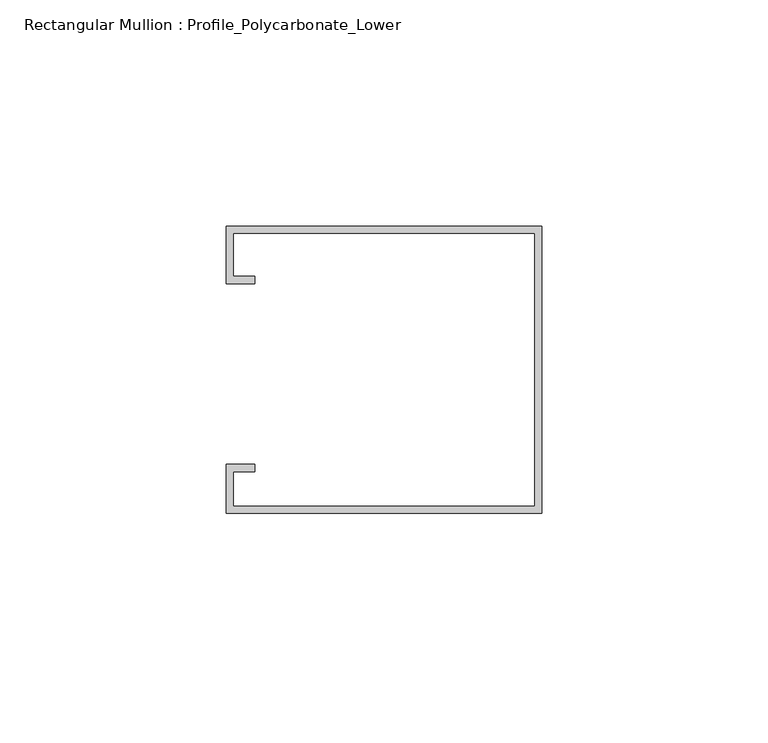
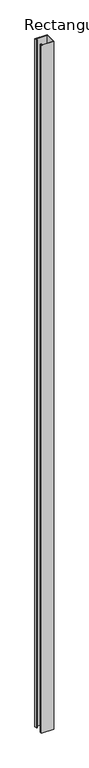
"""IFC4 building model written with IfcOpenShell, lengths in millimetres: member geometry, Rectangular Mullion : Profile_Polycarbonate_Lower."""

from ifc_helpers import new_model, si_unit, frame, origin, place, context, project, spatial, polyline, outline, extrude, source, transform, mapped, element, save


def rectangular_mullion_profile_polycarbonate_lower_04c0cb57(model_context):
    return source(origin(), model_context, "Body", "SweptSolid", [
        extrude(outline(polyline([(0.0, 32.7), (0.0, -30.8), (-69.85, -30.8), (-69.85, -20.0), (-63.5, -20.0), (-63.5, -21.5875), (-68.2625, -21.5875), (-68.2625, -29.2125), (-1.5875, -29.2125), (-1.5875, 31.1125), (-68.2625, 31.1125), (-68.2625, 21.5875), (-63.5, 21.5875), (-63.5, 20.0), (-69.85, 20.0), (-69.85, 32.7), (0.0, 32.7)])), frame((0.0, 0.0, -4143.375), z_axis=(0.0, 0.0, 1.0), x_axis=(1.0, 0.0, 0.0)), (0.0, 0.0, 1.0), 4143.375),
    ])


if __name__ == "__main__":
    model = new_model("IFC4")
    model_context = context("Model", 3, world=origin())
    ifc_project = project(units=[si_unit("LENGTHUNIT", "METRE", prefix="MILLI")], contexts=[model_context])
    site = spatial("IfcSite", under=ifc_project)
    building = spatial("IfcBuilding", under=site)
    placement = place(None, origin())
    rectangular_mullion_profile_polycarbonate_lower_shape = rectangular_mullion_profile_polycarbonate_lower_04c0cb57(model_context)
    element("IfcMember", 1, ObjectType="Rectangular Mullion : Profile_Polycarbonate_Lower", at=placement, inside=building, context=model_context, shape_type="MappedRepresentation", body=[
        mapped(rectangular_mullion_profile_polycarbonate_lower_shape, transform((0.0, 0.0, 0.0), x_axis=(1.0, 0.0, 0.0), y_axis=(0.0, 1.0, 0.0), z_axis=(0.0, 0.0, 1.0))),
    ])
    save(model, "model.ifc")

# Revit data of these elements
# Project information
#   Project Issue Date = "07/20/2015"
#   Project Status = "Project Status"
#   Client Name = "Xcel"
#   Project Address = "Enter address here"
#   Project Name = "Xcel Sports Complex"
#   Project Number = "Project Number"
# Type "Rectangular Mullion : Profile_Polycarbonate_Lower"
#   built-in parameter 1007322 = 0.208333 (stored number, unit not read)
#   built-in parameter 1007321 = 0 (stored number, unit not read)
#   built-in parameter 1007320 = 0.00520833 (stored number, unit not read)
